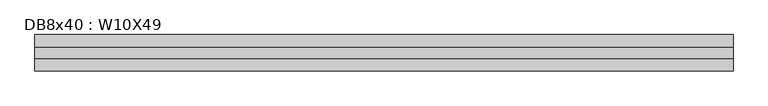
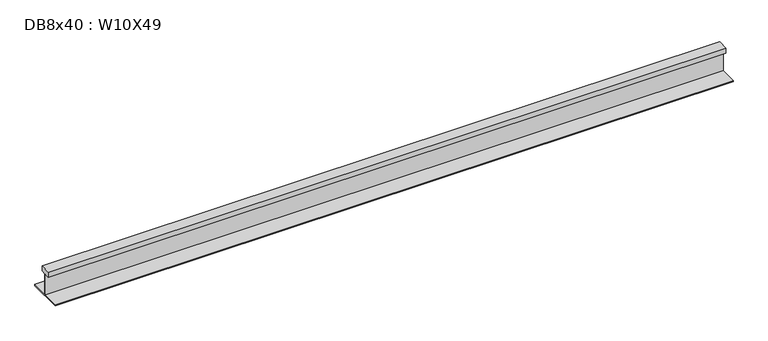
"""IFC4 building model written with IfcOpenShell, lengths in millimetres: beam geometry, DB8x40 : W10X49."""

from ifc_helpers import new_model, si_unit, frame, origin, place, context, project, spatial, polyline, outline, extrude, source, transform, mapped, element, save


def db8x40_w10x49_c5aa9a1a(model_context):
    return source(origin(), model_context, "Body", "SweptSolid", [
        extrude(outline(polyline([(38.1, 144.3355), (38.1, 106.2355), (2.921, 106.2355), (2.921, -49.53), (127.0, -49.53), (127.0, -59.182), (-127.0, -59.182), (-127.0, -49.53), (-2.921, -49.53), (-2.921, 106.2355), (-38.1, 106.2355), (-38.1, 144.3355), (38.1, 144.3355)])), frame((-2451.608, 0.0, 0.0), z_axis=(1.0, 0.0, 0.0), x_axis=(0.0, 1.0, 0.0)), (0.0, 0.0, 1.0), 4880.737),
    ])


if __name__ == "__main__":
    model = new_model("IFC4")
    model_context = context("Model", 3, world=origin())
    ifc_project = project(units=[si_unit("LENGTHUNIT", "METRE", prefix="MILLI")], contexts=[model_context])
    site = spatial("IfcSite", under=ifc_project)
    building = spatial("IfcBuilding", under=site)
    placement = place(None, origin())
    db8x40_w10x49_shape = db8x40_w10x49_c5aa9a1a(model_context)
    element("IfcBeam", 1, ObjectType="DB8x40 : W10X49", at=placement, inside=building, context=model_context, shape_type="MappedRepresentation", body=[
        mapped(db8x40_w10x49_shape, transform((0.0, 0.0, 0.0), x_axis=(1.0, 0.0, 0.0), y_axis=(0.0, 1.0, 0.0), z_axis=(0.0, 0.0, 1.0))),
    ])
    save(model, "model.ifc")

# Revit data of these elements
# Type "DB8x40 : W10X49"
#   Assembly Code = "B10"
#   W = 53
#   Length [instance default] = 5' - 0"
#   bf = 0' - 10"
#   d = 1' - 0.1"
#   k = 0' - 1 3/8"
#   k2 = 0' - 0.8"
#   tf = 0' - 0.575"
#   tw = 0' - 0.345"
#   A = 0.108333 SF
#   Structural Material [instance default] = Steel ASTM A992
# Element 1 (IfcBeam, "DB8x40 : W10X49")
#   Materials on its faces: "Steel ASTM A992"
# Materials
#   "Steel ASTM A992": class "Metal", colour RGB 199 199 199, transparency 0, Description = "Structural steel 50ksi", Cost = 0
